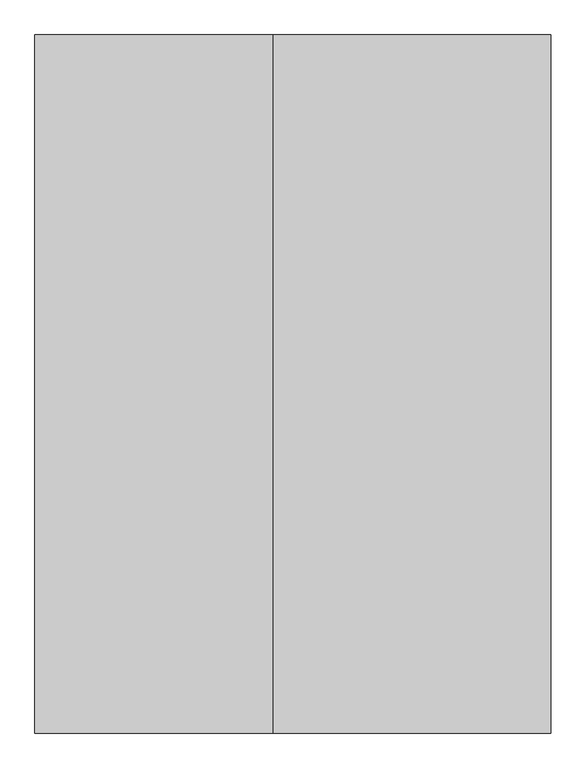
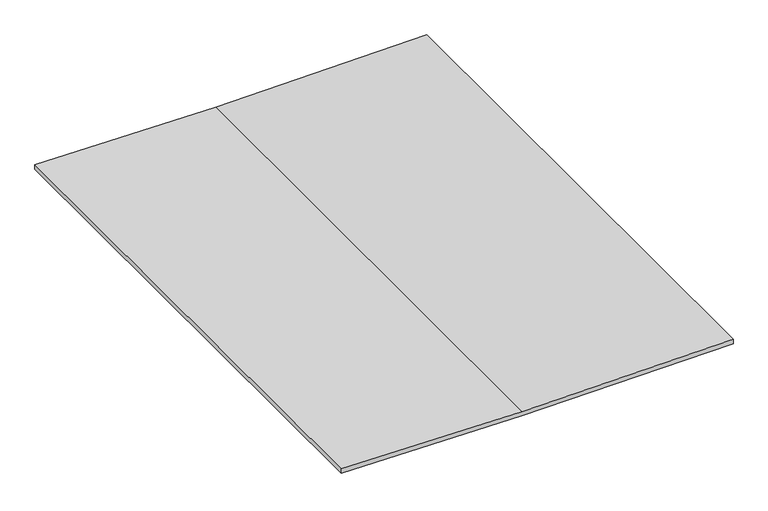
"""IFC4 building model written with IfcOpenShell, lengths in millimetres: proxy geometry, COVER BOARD002 14707 : COVER BOARD002 14707."""

import ifcopenshell
import ifcopenshell.guid

model = None  # the IFC model being written
_history = None  # IfcOwnerHistory: only IFC2X3 demands one
_inside = {}  # id of a spatial element -> (the spatial element, [elements in it])
_under = {}  # id of a project, library or spatial element -> (it, [spatial elements below it])
_declared = {}  # id of a project -> (the project, [libraries it declares])
_typed = {}  # id of a type object -> (the type object, [elements of that type])
_made_of = {}  # id of a material, layer set ... -> (it, [elements and type objects made of it])


def new_model(schema):
    """Start an empty IFC model of exactly this schema.

    Asked for "IFC4X3", IfcOpenShell would pick the latest addendum, in which some entities
    have other attributes; the version numbers below select the first issue.
    IFC2X3 requires an IfcOwnerHistory on every rooted entity: one is made here for all.
    """
    global model, _history
    if schema == "IFC4X3":
        model = ifcopenshell.file(schema_version=(4, 3, 0, 0))
    else:
        model = ifcopenshell.file(schema=schema)
    _inside.clear()
    _under.clear()
    _declared.clear()
    _typed.clear()
    _made_of.clear()
    _history = None
    if model.schema == "IFC2X3":
        org = make("IfcOrganization", Name="unknown")
        user = make(
            "IfcPersonAndOrganization",
            ThePerson=make("IfcPerson", FamilyName="unknown"),
            TheOrganization=org,
        )
        app = make(
            "IfcApplication",
            ApplicationDeveloper=org,
            Version="unknown",
            ApplicationFullName="unknown",
            ApplicationIdentifier="unknown",
        )
        _history = make(
            "IfcOwnerHistory",
            OwningUser=user,
            OwningApplication=app,
            ChangeAction="ADDED",
            CreationDate=0,
        )
    return model


def make(cls, **values):
    """One entity of the class cls with the attributes given. An attribute that is None is left unset."""
    return model.create_entity(
        cls, **{name: value for name, value in values.items() if value is not None}
    )


def rooted(cls, **values):
    """An entity with a GlobalId (a new one), such as an element, a storey or a relation."""
    return make(cls, GlobalId=ifcopenshell.guid.new(), OwnerHistory=_history, **values)


def si_unit(unit_type, name, prefix=None):
    """IfcSIUnit, for example si_unit("LENGTHUNIT", "METRE", prefix="MILLI")."""
    return make("IfcSIUnit", UnitType=unit_type, Prefix=prefix, Name=name)


def assignment(units):
    """IfcUnitAssignment: the units of a project."""
    return None if units is None else make("IfcUnitAssignment", Units=units)


def point(xyz):
    """IfcCartesianPoint."""
    return None if xyz is None else make("IfcCartesianPoint", Coordinates=xyz)


def direction(xyz):
    """IfcDirection."""
    return None if xyz is None else make("IfcDirection", DirectionRatios=xyz)


def frame(location, z_axis=None, x_axis=None):
    """IfcAxis2Placement3D, a coordinate frame: its origin and axes. An axis left out is left unset."""
    return make(
        "IfcAxis2Placement3D",
        Location=point(location),
        Axis=direction(z_axis),
        RefDirection=direction(x_axis),
    )


def origin():
    """The frame at (0, 0, 0) with its axes left unset."""
    return frame((0.0, 0.0, 0.0))


def place(relative_to, where):
    """IfcLocalPlacement: puts the frame where relative to a parent placement (None: the world)."""
    return make(
        "IfcLocalPlacement", PlacementRelTo=relative_to, RelativePlacement=where
    )


def context(
    kind, dimensions, precision=None, world=None, true_north=None, identifier=None
):
    """IfcGeometricRepresentationContext, for example the 3D "Model" context."""
    return make(
        "IfcGeometricRepresentationContext",
        ContextIdentifier=identifier,
        ContextType=kind,
        CoordinateSpaceDimension=dimensions,
        Precision=precision,
        WorldCoordinateSystem=world,
        TrueNorth=true_north,
    )


def project(units=None, contexts=None):
    """IfcProject with its units and contexts."""
    return rooted(
        "IfcProject",
        Name="project",
        RepresentationContexts=contexts,
        UnitsInContext=assignment(units),
    )


def spatial(cls, under=None, at=None, **own):
    """A site, building, storey or space (cls), placed at a placement, below another one or the project."""
    s = rooted(cls, ObjectPlacement=at, **own)
    if under is not None:
        _under.setdefault(under.id(), (under, []))[1].append(s)
    return s


def polyline(points):
    """IfcPolyline through the points."""
    return make("IfcPolyline", Points=[point(p) for p in points])


def outline(outer, holes=None, kind="AREA"):
    """IfcArbitraryClosedProfileDef: a profile drawn as a closed curve; with holes, ...WithVoids."""
    if holes is None:
        return make("IfcArbitraryClosedProfileDef", ProfileType=kind, OuterCurve=outer)
    return make(
        "IfcArbitraryProfileDefWithVoids",
        ProfileType=kind,
        OuterCurve=outer,
        InnerCurves=holes,
    )


def extrude(swept, where, along, depth):
    """IfcExtrudedAreaSolid: the profile swept, set in the frame where, extruded along a direction by depth."""
    return make(
        "IfcExtrudedAreaSolid",
        SweptArea=swept,
        Position=where,
        ExtrudedDirection=direction(along),
        Depth=depth,
    )


def shape(context_of_items, identifier, shape_type, items):
    """IfcShapeRepresentation: the items that make up one representation, for example the "Body"."""
    return make(
        "IfcShapeRepresentation",
        ContextOfItems=context_of_items,
        RepresentationIdentifier=identifier,
        RepresentationType=shape_type,
        Items=items,
    )


def source(mapping_origin, context_of_items, identifier, shape_type, items):
    """IfcRepresentationMap: a shape defined once, which mapped items show again and again."""
    return make(
        "IfcRepresentationMap",
        MappingOrigin=mapping_origin,
        MappedRepresentation=shape(context_of_items, identifier, shape_type, items),
    )


def transform(
    local_origin,
    x_axis=None,
    y_axis=None,
    z_axis=None,
    scale=None,
    scale2=None,
    scale3=None,
    uniform=True,
):
    """IfcCartesianTransformationOperator3D, or its non-uniform kind. x_axis, y_axis, z_axis: its Axis1, 2, 3."""
    if uniform:
        return make(
            "IfcCartesianTransformationOperator3D",
            Axis1=direction(x_axis),
            Axis2=direction(y_axis),
            LocalOrigin=point(local_origin),
            Scale=scale,
            Axis3=direction(z_axis),
        )
    return make(
        "IfcCartesianTransformationOperator3DnonUniform",
        Axis1=direction(x_axis),
        Axis2=direction(y_axis),
        LocalOrigin=point(local_origin),
        Scale=scale,
        Axis3=direction(z_axis),
        Scale2=scale2,
        Scale3=scale3,
    )


def mapped(mapping_source, mapping_target):
    """IfcMappedItem: shows the shape of a source again, moved by a transform."""
    return make(
        "IfcMappedItem", MappingSource=mapping_source, MappingTarget=mapping_target
    )


def made_of(thing, what):
    """Note that an element or type object is made of a material, layer set ...; save() writes the relation."""
    if what is not None:
        _made_of.setdefault(what.id(), (what, []))[1].append(thing)
    return thing


def element(
    cls,
    number,
    at=None,
    inside=None,
    cuts=None,
    type_object=None,
    material=None,
    context=None,
    identifier="Body",
    shape_type=None,
    held_by="IfcProductDefinitionShape",
    body=None,
    shapes=None,
    **own,
):
    """One element of the class cls, such as IfcWall. Its Tag is "e" and its number.

    at: its placement. inside: the storey or other place that contains it. cuts: it is an
    opening in that element (IfcRelVoidsElement). A single representation is given by context,
    identifier, shape_type and body (its items); several are given by shapes. held_by: the class
    of the entity that holds the representations. save() writes the other relations.
    """
    e = rooted(cls, Tag="e%d" % number, ObjectPlacement=at, **own)
    if body is not None:
        shapes = [shape(context, identifier, shape_type, body)]
    if shapes is not None:
        e.Representation = make(held_by, Representations=shapes)
    if inside is not None:
        _inside.setdefault(inside.id(), (inside, []))[1].append(e)
    if cuts is not None:
        rooted(
            "IfcRelVoidsElement", RelatingBuildingElement=cuts, RelatedOpeningElement=e
        )
    if type_object is not None:
        _typed.setdefault(type_object.id(), (type_object, []))[1].append(e)
    return made_of(e, material)


def aggregate(whole, parts):
    """IfcRelAggregates: a whole, such as a stair, and the parts it consists of."""
    return rooted("IfcRelAggregates", RelatingObject=whole, RelatedObjects=parts)


def save(model, path):
    """Write the relations noted so far, then the file.

    IfcRelAggregates (storeys below a building ...), IfcRelContainedInSpatialStructure (elements
    in a storey), IfcRelDefinesByType, IfcRelAssociatesMaterial and IfcRelDeclares: one each for
    every whole, place, type object, material and project.
    """
    for whole, parts in _under.values():
        aggregate(whole, parts)
    for where, things in _inside.values():
        rooted(
            "IfcRelContainedInSpatialStructure",
            RelatedElements=things,
            RelatingStructure=where,
        )
    for kind, things in _typed.values():
        rooted("IfcRelDefinesByType", RelatedObjects=things, RelatingType=kind)
    for what, things in _made_of.values():
        rooted("IfcRelAssociatesMaterial", RelatedObjects=things, RelatingMaterial=what)
    for by, libraries in _declared.values():
        rooted("IfcRelDeclares", RelatingContext=by, RelatedDefinitions=libraries)
    model.write(path)


def generic_models_e83da0d9(model_context):
    return source(origin(), model_context, "Body", "SweptSolid", [
        extrude(outline(polyline([(40228.1021556, -1886.5629484), (40237.9000089, -2567.3737014), (40220.5682898, -2567.3737014), (40210.7704365, -1886.5629484), (40220.5682898, -1090.0815411), (40237.9000089, -1090.0815411), (40228.1021556, -1886.5629484)])), frame((0.0, 1000.0, 0.0), z_axis=(0.0, 1.0, 0.0), x_axis=(0.0, 0.0, 1.0)), (0.0, 0.0, 1.0), 2000.0),
    ])


if __name__ == "__main__":
    model = new_model("IFC4")
    model_context = context("Model", 3, world=origin())
    ifc_project = project(units=[si_unit("LENGTHUNIT", "METRE", prefix="MILLI")], contexts=[model_context])
    site = spatial("IfcSite", under=ifc_project)
    building = spatial("IfcBuilding", under=site)
    placement = place(None, origin())
    generic_models_shape = generic_models_e83da0d9(model_context)
    element("IfcBuildingElementProxy", 1, Name="COVER BOARD002 14707 : COVER BOARD002 14707", ObjectType="COVER BOARD002 14707 : COVER BOARD002 14707", at=placement, inside=building, context=model_context, shape_type="MappedRepresentation", body=[
        mapped(generic_models_shape, transform((0.0, 0.0, 0.0), x_axis=(1.0, 0.0, 0.0), y_axis=(0.0, 1.0, 0.0), z_axis=(0.0, 0.0, 1.0))),
    ])
    save(model, "model.ifc")

# Revit data of these elements
# Type "COVER BOARD002 14707 : COVER BOARD002 14707"
#   NameOverride = "COVER BOARD002"
# Element 1 (IfcBuildingElementProxy, "COVER BOARD002 14707 : COVER BOARD002 14707")
#   Materials on its faces: "CDX PLYWOOD - SEE STRUCTURAL DWGS"
# Materials
#   "CDX PLYWOOD - SEE STRUCTURAL DWGS": class "Unassigned", colour RGB 138 93 50, transparency 0, Cost = 0
